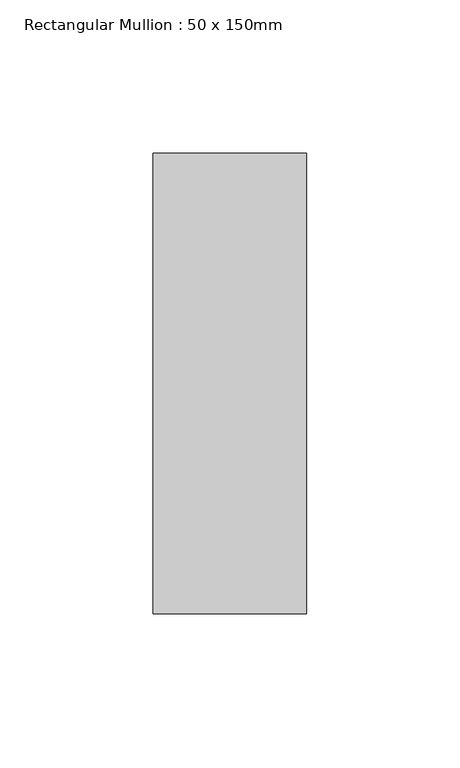
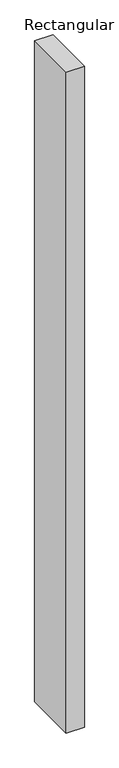
"""IFC4 building model written with IfcOpenShell, lengths in millimetres: member geometry, Rectangular Mullion : 50 x 150mm."""

from ifc_helpers import new_model, si_unit, frame, origin, place, context, project, spatial, polyline, outline, extrude, source, transform, mapped, element, save


def rectangular_mullion_50_x_150mm_6ba4331c(model_context):
    return source(origin(), model_context, "Body", "SweptSolid", [
        extrude(outline(polyline([(25.0, 75.0), (25.0, -75.0), (-25.0, -75.0), (-25.0, 75.0), (25.0, 75.0)])), frame((0.0, 0.0, -1923.3666669), z_axis=(0.0, 0.0, 1.0), x_axis=(1.0, 0.0, 0.0)), (0.0, 0.0, 1.0), 1923.3666669),
    ])


if __name__ == "__main__":
    model = new_model("IFC4")
    model_context = context("Model", 3, world=origin())
    ifc_project = project(units=[si_unit("LENGTHUNIT", "METRE", prefix="MILLI")], contexts=[model_context])
    site = spatial("IfcSite", under=ifc_project)
    building = spatial("IfcBuilding", under=site)
    placement = place(None, origin())
    rectangular_mullion_50_x_150mm_shape = rectangular_mullion_50_x_150mm_6ba4331c(model_context)
    element("IfcMember", 1, ObjectType="Rectangular Mullion : 50 x 150mm", at=placement, inside=building, context=model_context, shape_type="MappedRepresentation", body=[
        mapped(rectangular_mullion_50_x_150mm_shape, transform((0.0, 0.0, 0.0), x_axis=(1.0, 0.0, 0.0), y_axis=(0.0, 1.0, 0.0), z_axis=(0.0, 0.0, 1.0))),
    ])
    save(model, "model.ifc")

# Revit data of these elements
# Type "Rectangular Mullion : 50 x 150mm"
#   built-in parameter 1007304 = 0.492126 (stored number, unit not read)
#   built-in parameter 1007301 = 0.082021 (stored number, unit not read)
#   built-in parameter 1007300 = 0.082021 (stored number, unit not read)
# Element 1 (IfcMember, "Rectangular Mullion : 50 x 150mm")
#   Materials on its faces: "Metal - Aluminium"
# Materials
#   "Metal - Aluminium": class "Metal", colour RGB 247 247 247, transparency 0
